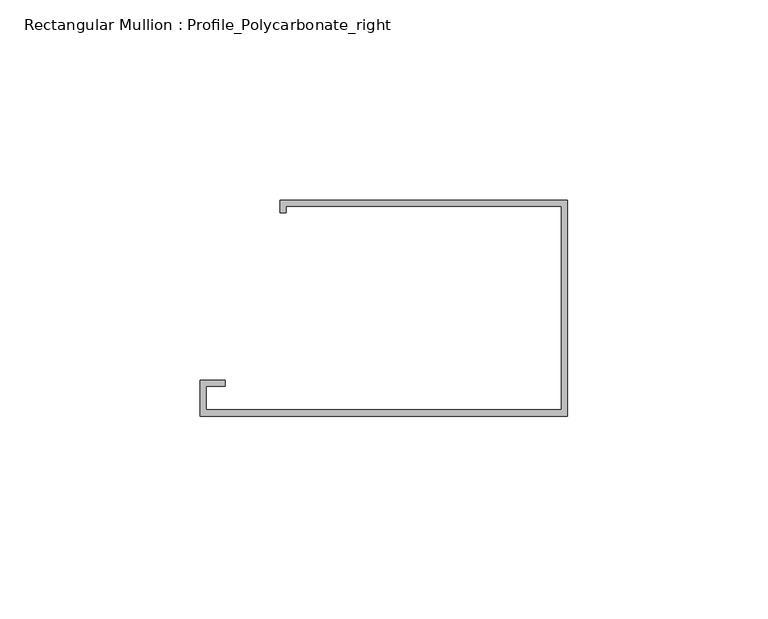
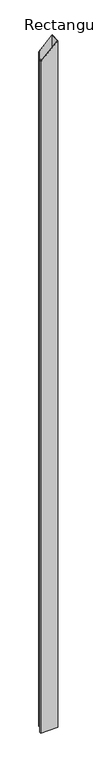
"""IFC4 building model written with IfcOpenShell, lengths in millimetres: member geometry, Rectangular Mullion : Profile_Polycarbonate_right."""

from ifc_helpers import new_model, si_unit, origin, place, context, project, spatial, faceted_brep, source, transform, mapped, element, save


def rectangular_mullion_profile_polycarbonate_right_756e7e87(model_context):
    return source(origin(), model_context, "Body", "Brep", [
        faceted_brep([(0.0, -28.984575, -3894.7989583), (-91.9988, -28.984575, -3894.7989583), (-91.9988, -19.992975, -3894.7989583), (-85.6488, -19.992975, -3894.7989583), (-85.6488, -21.580475, -3894.7989583), (-90.4113, -21.580475, -3894.7989583), (-90.4113, -27.397075, -3894.7989583), (-1.5875, -27.397075, -3894.7989583), (-1.5875, 23.428325, -3894.7989583), (-70.3961, 23.428325, -3894.7989583), (-70.3961, 21.840825, -3894.7989583), (-71.9836, 21.840825, -3894.7989583), (-71.9836, 25.015825, -3894.7989583), (0.0, 25.015825, -3894.7989583), (0.0, 25.015825, 0.0), (0.0, -28.984575, 0.0), (-71.9836, 25.015825, -69.046742), (-71.9836, 21.840825, -69.046742), (-70.3961, 21.840825, -67.5240104), (-70.3961, 23.428325, -67.5240104), (-1.5875, 23.428325, -1.5227316), (-1.5875, -27.397075, -1.5227316), (-90.4113, -27.397075, -86.7226105), (-90.4113, -21.580475, -86.7226105), (-85.6488, -21.580475, -82.1544157), (-85.6488, -19.992975, -82.1544157), (-91.9988, -19.992975, -88.2453421), (-91.9988, -28.984575, -88.2453421)], [[[0, 1, 2, 3, 4, 5, 6, 7, 8, 9, 10, 11, 12, 13]], [[14, 15, 0, 13]], [[16, 14, 13, 12]], [[17, 16, 12, 11]], [[18, 17, 11, 10]], [[19, 18, 10, 9]], [[20, 19, 9, 8]], [[21, 20, 8, 7]], [[22, 21, 7, 6]], [[23, 22, 6, 5]], [[24, 23, 5, 4]], [[25, 24, 4, 3]], [[26, 25, 3, 2]], [[27, 26, 2, 1]], [[15, 27, 1, 0]], [[15, 14, 16, 17, 18, 19, 20, 21, 22, 23, 24, 25, 26, 27]]]),
    ])


if __name__ == "__main__":
    model = new_model("IFC4")
    model_context = context("Model", 3, world=origin())
    ifc_project = project(units=[si_unit("LENGTHUNIT", "METRE", prefix="MILLI")], contexts=[model_context])
    site = spatial("IfcSite", under=ifc_project)
    building = spatial("IfcBuilding", under=site)
    placement = place(None, origin())
    rectangular_mullion_profile_polycarbonate_right_shape = rectangular_mullion_profile_polycarbonate_right_756e7e87(model_context)
    element("IfcMember", 1, ObjectType="Rectangular Mullion : Profile_Polycarbonate_right", at=placement, inside=building, context=model_context, shape_type="MappedRepresentation", body=[
        mapped(rectangular_mullion_profile_polycarbonate_right_shape, transform((0.0, 0.0, 0.0), x_axis=(1.0, 0.0, 0.0), y_axis=(0.0, 1.0, 0.0), z_axis=(0.0, 0.0, 1.0))),
    ])
    save(model, "model.ifc")

# Revit data of these elements
# Type "Rectangular Mullion : Profile_Polycarbonate_right"
#   built-in parameter 1007322 = 0.177167 (stored number, unit not read)
#   built-in parameter 1007321 = 0 (stored number, unit not read)
#   built-in parameter 1007320 = 0.00520833 (stored number, unit not read)
